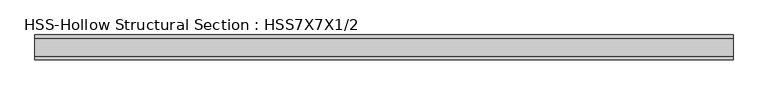
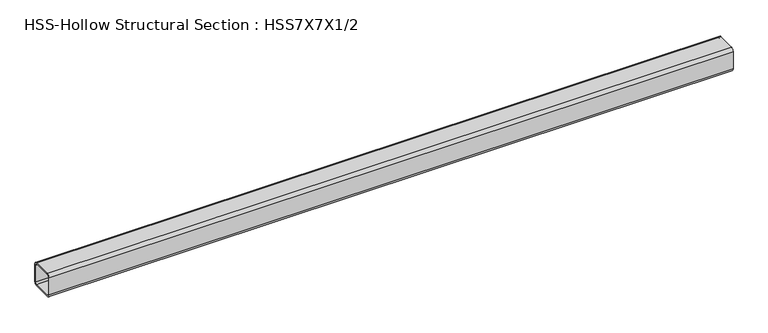
"""IFC4 building model written with IfcOpenShell, lengths in millimetres: member geometry, HSS-Hollow Structural Section : HSS7X7X1/2."""

from ifc_helpers import new_model, si_unit, point, frame, frame_2d, origin, place, context, project, spatial, polyline, circle_curve, trimmed, segment, composite_curve, outline, extrude, source, transform, mapped, element, save


def hss_hollow_structural_section_hss7x7x1_2_2d55a091(model_context):
    return source(origin(), model_context, "Body", "SweptSolid", [
        extrude(outline(composite_curve([segment(polyline([(88.9, 65.278), (88.9, -65.278)]), True, "CONTINUOUS"), segment(trimmed(circle_curve(frame_2d((65.278, -65.278)), 23.622), [point((88.9, -65.278))], [point((65.278, -88.9))], False, "CARTESIAN"), True, "CONTINUOUS"), segment(polyline([(65.278, -88.9), (-65.278, -88.9)]), True, "CONTINUOUS"), segment(trimmed(circle_curve(frame_2d((-65.278, -65.278)), 23.622), [point((-65.278, -88.9))], [point((-88.9, -65.278))], False, "CARTESIAN"), True, "CONTINUOUS"), segment(polyline([(-88.9, -65.278), (-88.9, 65.278)]), True, "CONTINUOUS"), segment(trimmed(circle_curve(frame_2d((-65.278, 65.278)), 23.622), [point((-88.9, 65.278))], [point((-65.278, 88.9))], False, "CARTESIAN"), True, "CONTINUOUS"), segment(polyline([(-65.278, 88.9), (65.278, 88.9)]), True, "CONTINUOUS"), segment(trimmed(circle_curve(frame_2d((65.278, 65.278)), 23.622), [point((65.278, 88.9))], [point((88.9, 65.278))], False, "CARTESIAN"), True, "CONTINUOUS")], self_intersect=False), holes=[composite_curve([segment(trimmed(circle_curve(frame_2d((-65.278, 65.278)), 11.811), [point((-65.278, 77.089))], [point((-77.089, 65.278))], True, "CARTESIAN"), True, "CONTINUOUS"), segment(polyline([(-77.089, 65.278), (-77.089, -65.278)]), True, "CONTINUOUS"), segment(trimmed(circle_curve(frame_2d((-65.278, -65.278)), 11.811), [point((-77.089, -65.278))], [point((-65.278, -77.089))], True, "CARTESIAN"), True, "CONTINUOUS"), segment(polyline([(-65.278, -77.089), (65.278, -77.089)]), True, "CONTINUOUS"), segment(trimmed(circle_curve(frame_2d((65.278, -65.278)), 11.811), [point((65.278, -77.089))], [point((77.089, -65.278))], True, "CARTESIAN"), True, "CONTINUOUS"), segment(polyline([(77.089, -65.278), (77.089, 65.278)]), True, "CONTINUOUS"), segment(trimmed(circle_curve(frame_2d((65.278, 65.278)), 11.811), [point((77.089, 65.278))], [point((65.278, 77.089))], True, "CARTESIAN"), True, "CONTINUOUS"), segment(polyline([(65.278, 77.089), (-65.278, 77.089)]), True, "CONTINUOUS")], self_intersect=False)]), frame((-2577.621329, 0.0, 0.0), z_axis=(1.0, 0.0, 0.0), x_axis=(0.0, 1.0, 0.0)), (0.0, 0.0, 1.0), 4993.3144287),
    ])


if __name__ == "__main__":
    model = new_model("IFC4")
    model_context = context("Model", 3, world=origin())
    ifc_project = project(units=[si_unit("LENGTHUNIT", "METRE", prefix="MILLI")], contexts=[model_context])
    site = spatial("IfcSite", under=ifc_project)
    building = spatial("IfcBuilding", under=site)
    placement = place(None, origin())
    hss_hollow_structural_section_hss7x7x1_2_shape = hss_hollow_structural_section_hss7x7x1_2_2d55a091(model_context)
    element("IfcMember", 1, ObjectType="HSS-Hollow Structural Section : HSS7X7X1/2", at=placement, inside=building, context=model_context, shape_type="MappedRepresentation", body=[
        mapped(hss_hollow_structural_section_hss7x7x1_2_shape, transform((0.0, 0.0, 0.0), x_axis=(1.0, 0.0, 0.0), y_axis=(0.0, 1.0, 0.0), z_axis=(0.0, 0.0, 1.0))),
    ])
    save(model, "model.ifc")

# Revit data of these elements
# Type "HSS-Hollow Structural Section : HSS7X7X1/2"
#   Assembly Code = "B10"
#   Shape = "Square"
#   W = 41.9
#   Ht = 0' - 7"
#   Length [instance default] = 5' - 0"
#   b = 0' - 7"
#   kr = 0' - 0.93"
#   t = 0' - 0.465"
#   A = 0.0805556 SF
#   Structural Material [instance default] = Steel ASTM A500, Grade B, Rectangular and Square
# Element 1 (IfcMember, "HSS-Hollow Structural Section : HSS7X7X1/2")
#   Materials on its faces: "Steel ASTM A500, Grade B, Rectangular and Square"
# Materials
#   "Steel ASTM A500, Grade B, Rectangular and Square": class "Metal", colour RGB 199 199 199, transparency 0, Description = "Carbon steel", Cost = 0
